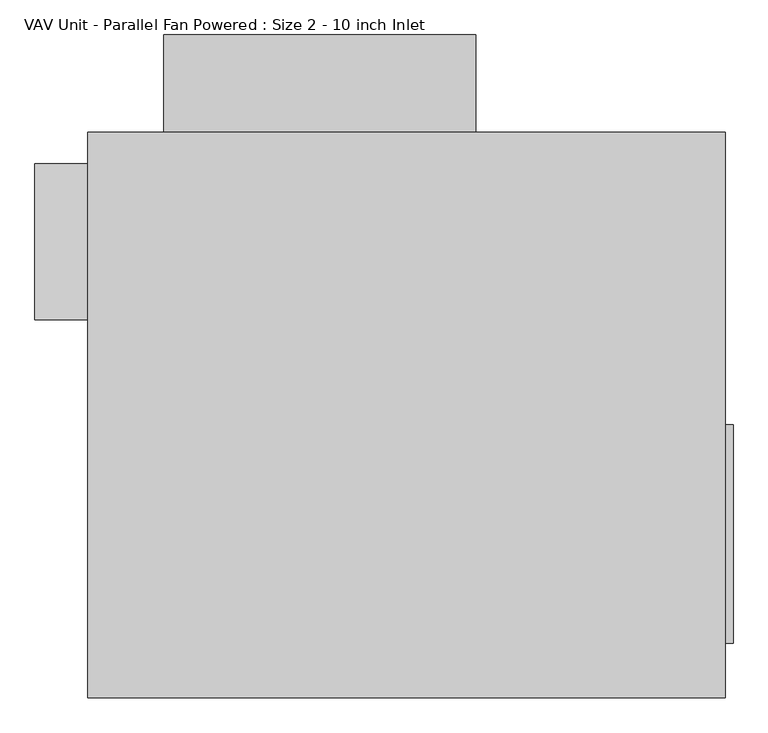
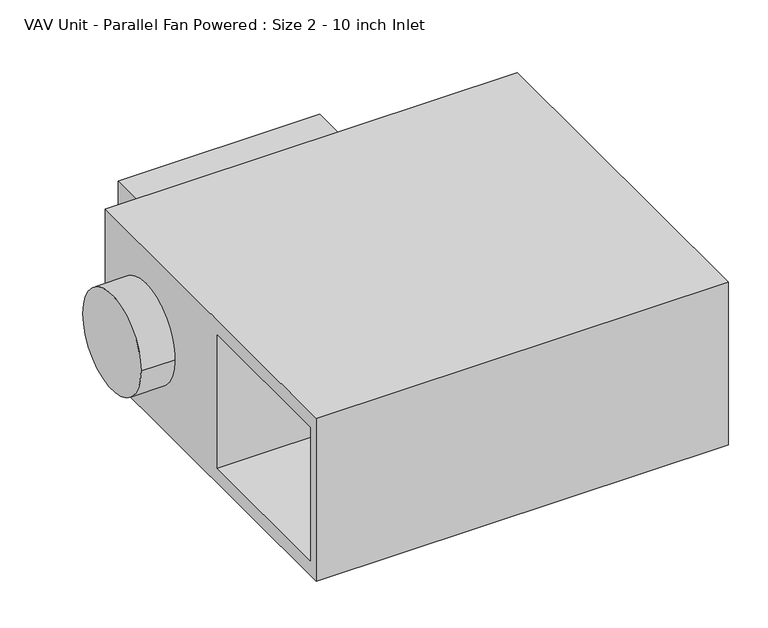
"""IFC4 building model written with IfcOpenShell, lengths in millimetres: proxy geometry, VAV Unit - Parallel Fan Powered : Size 2 - 10 inch Inlet."""

from ifc_helpers import new_model, si_unit, point, frame, frame_2d, origin, place, context, project, spatial, polyline, circle_curve, trimmed, segment, composite_curve, outline, extrude, faceted_brep, source, transform, mapped, element, save


def vav_unit_parallel_fan_powered_size_2_10_inch_inlet_b65b1531(model_context):
    return source(origin(), model_context, "Body", "SolidModel", [
        extrude(outline(polyline([(531.8125, -15.875), (531.8125, -371.475), (519.1125, -371.475), (519.1125, -15.875), (531.8125, -15.875)])), frame((0.0, 0.0, -139.7), z_axis=(0.0, 0.0, 1.0), x_axis=(1.0, 0.0, 0.0)), (0.0, 0.0, 1.0), 279.4),
        extrude(outline(polyline([(112.7125, 460.375), (-395.2875, 460.375), (-395.2875, 619.125), (112.7125, 619.125), (112.7125, 460.375)])), frame((0.0, 0.0, -152.4), z_axis=(0.0, 0.0, 1.0), x_axis=(1.0, 0.0, 0.0)), (0.0, 0.0, 1.0), 304.8),
        extrude(outline(composite_curve([segment(trimmed(circle_curve(frame_2d((282.575, 0.0)), 127.0), [point((155.575, 0.0))], [point((409.575, 0.0))], False, "CARTESIAN"), True, "CONTINUOUS"), segment(trimmed(circle_curve(frame_2d((282.575, 0.0)), 127.0), [point((409.575, 0.0))], [point((155.575, 0.0))], False, "CARTESIAN"), True, "CONTINUOUS")], self_intersect=False)), frame((-604.8375, 0.0, 0.0), z_axis=(1.0, 0.0, 0.0), x_axis=(0.0, 1.0, 0.0)), (0.0, 0.0, 1.0), 85.725),
        faceted_brep([(519.1125, 460.375, 217.4875), (-519.1125, 460.375, 217.4875), (-519.1125, -460.375, 217.4875), (519.1125, -460.375, 217.4875), (519.1125, 460.375, -217.4875), (519.1125, -460.375, -217.4875), (-519.1125, -460.375, -217.4875), (-519.1125, 460.375, -217.4875), (-519.1125, -434.975, 177.8), (-519.1125, -434.975, -177.8), (-519.1125, -28.575, -177.8), (-519.1125, -28.575, 177.8), (0.0, -434.975, 177.8), (0.0, -28.575, 177.8), (0.0, -28.575, -177.8), (0.0, -434.975, -177.8)], [[[0, 1, 2, 3]], [[4, 5, 6, 7]], [[1, 0, 4, 7]], [[2, 1, 7, 6], [8, 9, 10, 11]], [[3, 2, 6, 5]], [[0, 3, 5, 4]], [[12, 13, 14, 15]], [[12, 15, 9, 8]], [[15, 14, 10, 9]], [[14, 13, 11, 10]], [[13, 12, 8, 11]]]),
    ])


if __name__ == "__main__":
    model = new_model("IFC4")
    model_context = context("Model", 3, world=origin())
    ifc_project = project(units=[si_unit("LENGTHUNIT", "METRE", prefix="MILLI")], contexts=[model_context])
    site = spatial("IfcSite", under=ifc_project)
    building = spatial("IfcBuilding", under=site)
    placement = place(None, origin())
    vav_unit_parallel_fan_powered_size_2_10_inch_inlet_shape = vav_unit_parallel_fan_powered_size_2_10_inch_inlet_b65b1531(model_context)
    element("IfcBuildingElementProxy", 1, Name="VAV Unit - Parallel Fan Powered : Size 2 - 10 inch Inlet", ObjectType="VAV Unit - Parallel Fan Powered : Size 2 - 10 inch Inlet", at=placement, inside=building, context=model_context, shape_type="MappedRepresentation", body=[
        mapped(vav_unit_parallel_fan_powered_size_2_10_inch_inlet_shape, transform((0.0, 0.0, 0.0), x_axis=(1.0, 0.0, 0.0), y_axis=(0.0, 1.0, 0.0), z_axis=(0.0, 0.0, 1.0))),
    ])
    save(model, "model.ifc")

# Revit data of these elements
# Type "VAV Unit - Parallel Fan Powered : Size 2 - 10 inch Inlet"
#   Width2 = 1' - 2"
#   Voltage = 120 V
#   UnitWidth = 3' - 4 7/8"
#   UnitHeight = 3' - 0 1/4"
#   UnitDepth = 1' - 5 1/8"
#   SupplyConnectorWidth = 1' - 2"
#   SupplyConnectorVerticalOffset = 0' - 2 1/8"
#   SupplyConnectorLength = 0' - 0 1/2"
#   SupplyConnectorHorizontalOffset = 0' - 3 1/2"
#   SupplyConnectorDepth = 0' - 11"
#   SupplyAirConnectorCenterOffset = 0' - 10 1/2"
#   PrimaryToSupplyRatio [instance default] = 0.2
#   PrimaryAirOffset = 0' - 7"
#   PrimaryAirFlow [instance default] = 280 CFM
#   PrimaryAirConnectorVerticalOffset = 0' - 8 9/16"
#   PrimaryAirConnectorRadius = 0' - 5"
#   PrimaryAirConnectorLength = 0' - 3 3/8"
#   PrimaryAirConnectorDiameter = 0' - 10"
#   PrimaryAirConnectorCenterOffset = 0' - 7"
#   Pressure Drop [instance default] = 0.01 in-wg
#   InducedAirInletWidth = 1' - 4"
#   InducedAirInletDepth = 1' - 2"
#   InducedAirConnectorHorizontalOffset = 0' - 1"
#   InducedAirConnectorCenterOffset = 0' - 9"
#   Height2 = 0' - 11"
#   ElectricalConnectionBoxWidth = 1' - 8"
#   ElectricalConnectionBoxOffset = 0' - 4 7/8"
#   ElectricalConnectionBoxHeight = 0' - 6 1/4"
#   ElectricalConnectionBoxDepth = 1' - 0"
#   SupplyAirFlow [instance default] = 1400 CFM
#   Apparent Load = 542 VA
#   SupplyAirConnectorIndex = 2
#   PrimaryAirConnectorIndex = 1
#   Number of Poles = 1
#   InducedAirConnectorIndex = 3
#   VAV Material = none
#   Load Classification = Cooling
#   Default Elevation = 0
#   Assembly Code = ""
